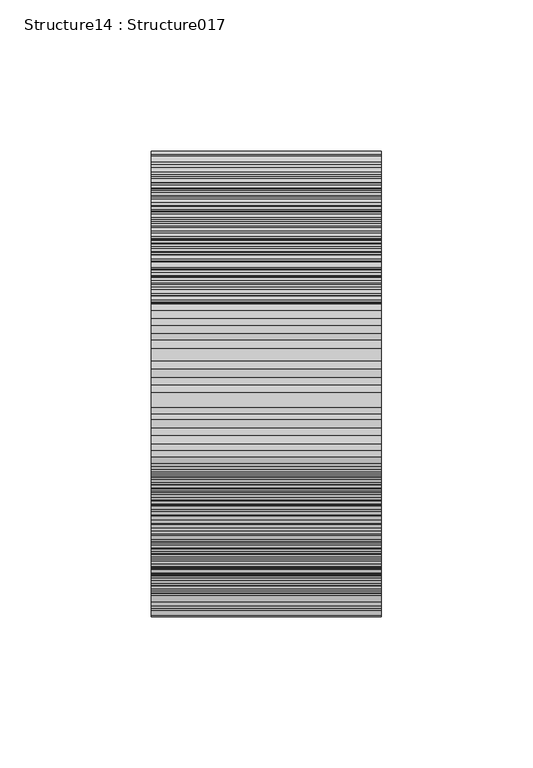
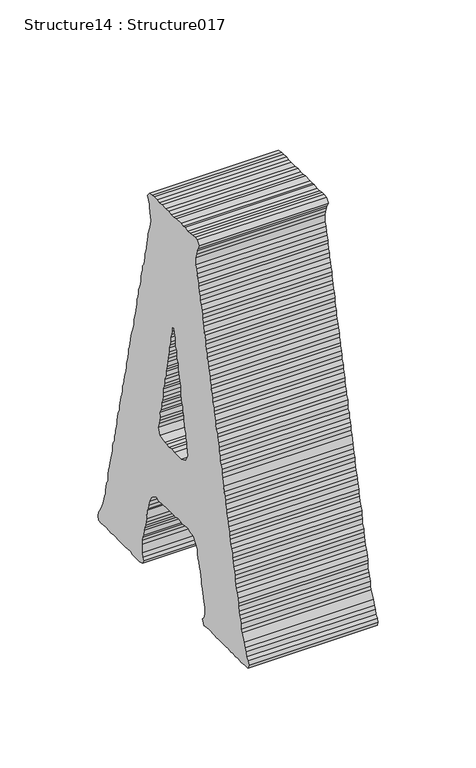
"""IFC4 building model written with IfcOpenShell, lengths in millimetres: proxy geometry, Structure14 : Structure017."""

from ifc_helpers import new_model, si_unit, frame, origin, place, context, project, spatial, polyline, outline, extrude, source, transform, mapped, element, save


def structure14_structure017_488298b9(model_context):
    return source(origin(), model_context, "Body", "SweptSolid", [
        extrude(outline(polyline([(2.1653931, 0.0), (4.9551582, -1.2411193), (7.1205514, -1.549493), (9.8959144, -1.8578666), (12.3790002, -2.7906123), (14.2258535, -3.0981388), (17.0249376, -4.0215654), (19.4987044, -4.0215654), (22.2740675, -4.9543111), (24.4394606, -5.5710584), (27.2292257, -6.1861114), (29.3937717, -6.8121777), (31.8616083, -7.1197042), (33.7101559, -8.0431309), (36.8159193, -8.3557404), (38.9813125, -8.3557404), (41.7583699, -8.9758765), (43.3112516, -9.9009975), (46.4093904, -10.5211336), (48.2664099, -11.1412697), (50.7384823, -11.758017), (53.207166, -11.758017), (55.371712, -12.3781531), (58.1614771, -13.3015797), (60.6428686, -14.2300895), (63.419926, -14.2300895), (65.2676265, -15.1585992), (68.3750842, -15.7795824), (70.2219375, -15.7795824), (72.7041762, -16.7080922), (75.1770958, -17.0198546), (77.9524588, -17.6366019), (80.1322541, -18.5642645), (84.4621932, -18.5642645), (86.9291825, -17.9432812), (89.4029494, -17.3231452), (91.2591217, -16.3997185), (93.7311941, -15.1585992), (96.2142799, -17.3231452), (96.5226536, -19.4885383), (96.5226536, -21.6581674), (95.9109893, -24.4428494), (95.9109893, -26.9149218), (96.5226536, -29.7012982), (96.2142799, -31.5532346), (96.5226536, -33.7237108), (96.5226536, -38.673786), (95.9109893, -41.1407754), (95.9109893, -43.6187781), (96.5226536, -46.4085432), (96.2142799, -49.1847535), (96.2142799, -53.2063189), (95.9109893, -55.996084), (96.5226536, -58.16063), (96.5226536, -60.9410761), (96.2142799, -63.1064692), (95.9109893, -65.8911513), (93.4245148, -67.7490179), (91.2591217, -66.5172176), (89.0945757, -65.8911513), (87.2375562, -65.584472), (84.4621932, -64.9634887), (79.8094783, -64.0392149), (77.6457795, -64.6610453), (74.8687221, -65.2710152), (69.9135639, -67.1280347), (68.3750842, -67.1280347), (65.5853191, -67.7490179), (63.1166354, -68.369154), (60.3268703, -68.6775277), (57.8437845, -69.2934278), (55.371712, -70.538783), (53.5155397, -70.538783), (50.7384823, -70.8429208), (48.2664099, -71.4630569), (46.4093904, -72.6990931), (43.6196253, -72.6990931), (41.1467056, -73.6276028), (38.9813125, -74.2477389), (36.5134759, -74.2477389), (33.7101559, -74.8636391), (31.2507912, -75.792996), (29.085398, -76.7215057), (27.2292257, -77.028185), (24.4394606, -77.3416418), (22.2740675, -78.2693043), (19.4987044, -78.2693043), (17.0249376, -79.1935782), (14.8510727, -79.5061878), (12.0748624, -80.1263238), (7.7322156, -81.6715809), (4.9551582, -81.6715809), (2.7906123, -82.291717), (0.3176926, -82.90677), (-2.4720725, -84.1478893), (-4.3282448, -84.4562629), (-6.8020116, -85.0721631), (-9.283403, -85.3847727), (-12.0604605, -86.3132824), (-13.9217158, -86.9283354), (-16.7063979, -86.9283354), (-19.4826081, -87.8568451), (-21.3438635, -88.1703019), (-24.1344758, -89.0937285), (-26.5929933, -89.4063381), (-29.0752319, -89.7147118), (-30.9322514, -90.3348478), (-33.4136429, -91.2582745), (-36.4982268, -91.5717313), (-38.9711464, -92.1918673), (-40.5240281, -93.115294), (-43.3002383, -93.115294), (-46.0908506, -93.7362772), (-48.2553966, -94.6605511), (-51.0409258, -95.2806871), (-52.9021812, -95.9008232), (-55.0531722, -96.5167233), (-57.5354109, -96.5167233), (-60.6327025, -97.7586898), (-63.1013862, -98.3737428), (-65.2794871, -98.6821165), (-67.7524067, -98.6821165), (-69.6094262, -99.3022526), (-72.6931629, -100.2349982), (-74.5501824, -100.539136), (-77.032421, -101.4718816), (-79.8128671, -101.4718816), (-81.9782603, -102.7036819), (-84.1428062, -103.323818), (-86.6106428, -103.323818), (-89.386853, -103.9439541), (-92.1910202, -104.8673807), (-94.3420113, -105.493447), (-96.2032666, -106.1093472), (-98.9887958, -106.4168737), (-101.4617155, -107.3453834), (-104.2514806, -107.9655195), (-106.7193172, -107.9655195), (-108.8982652, -108.2696573), (-111.0492563, -109.5150125), (-113.8390214, -110.1309126), (-116.311941, -110.74766), (-118.476487, -110.74766), (-120.6503519, -111.6804056), (-125.8994818, -113.2239683), (-128.0784298, -114.147395), (-129.9261303, -115.0809878), (-132.7116595, -116.9329242), (-134.2560694, -117.5589905), (-137.0314325, -118.4824172), (-139.2061446, -117.8656699), (-139.5136711, -114.7692254), (-139.2061446, -112.9113588), (-138.8884519, -110.1309126), (-139.5136711, -107.6588402), (-139.5136711, -104.8673807), (-138.8884519, -102.3953083), (-138.8884519, -100.2349982), (-139.2061446, -97.7586898), (-139.2061446, -95.5932967), (-139.5136711, -92.4951579), (-139.5136711, -90.3348478), (-139.2061446, -87.8568451), (-138.8884519, -85.0721631), (-139.5136711, -82.90677), (-139.5136711, -75.792996), (-138.8884519, -73.0066196), (-136.7374609, -71.7714306), (-134.8762055, -72.6990931), (-132.4083689, -73.3192292), (-127.1363652, -73.3192292), (-124.6634456, -73.3192292), (-122.4988996, -72.6990931), (-120.6503519, -71.7714306), (-117.5437413, -71.4630569), (-115.3791954, -70.8429208), (-113.2138022, -69.9135639), (-111.0492563, -69.2934278), (-108.5805725, -68.6775277), (-103.0145972, -68.0607803), (-101.4617155, -67.4414914), (-98.9887958, -66.5172176), (-95.8957401, -65.8911513), (-92.8018373, -64.3475886), (-90.9405819, -62.1830426), (-89.0928814, -58.7773773), (-89.7045457, -56.3044577), (-89.7045457, -51.3543825), (-89.386853, -48.2604796), (-89.386853, -41.7668417), (-89.7045457, -38.9762294), (-89.0928814, -36.8167666), (-89.386853, -34.3429997), (-89.7045457, -31.8666914), (-89.386853, -29.7012982), (-89.0928814, -26.6082425), (-89.7045457, -24.7512231), (-90.6372913, -21.04142), (-92.4943108, -19.1801646), (-95.8957401, -16.7080922), (-98.6719504, -16.7080922), (-101.4617155, -16.0862617), (-103.0145972, -15.1585992), (-106.0991811, -14.8544614), (-107.9697554, -13.6141893), (-110.7459657, -12.9982891), (-112.6029851, -12.6865267), (-115.0759048, -12.6865267), (-117.5437413, -11.4445602), (-120.0302159, -11.1412697), (-122.4988996, -10.8337432), (-124.6634456, -9.9009975), (-127.7607372, -8.9758765), (-131.7831498, -9.2800143), (-134.8762055, -10.208524), (-136.4206154, -11.758017), (-139.5136711, -9.9009975), (-139.2061446, -7.1197042), (-138.8884519, -4.6425487), (-138.8884519, 0.3075265), (-139.2061446, 2.7804461), (-139.2061446, 5.2525186), (-138.8884519, 7.4229948), (-139.2061446, 9.5875408), (-139.2061446, 12.6805965), (-138.8884519, 14.5333801), (-139.2061446, 17.6315188), (-138.8884519, 19.4876911), (-139.5136711, 21.9648467), (-138.8884519, 24.74614), (-139.5136711, 27.5316692), (-139.2061446, 29.6962152), (-138.8884519, 32.1733707), (-138.8884519, 34.6420544), (-136.4206154, 35.5748001), (-134.2560694, 34.954664), (-132.7116595, 33.405171), (-129.9261303, 32.790118), (-128.0784298, 31.8616083), (-125.2742626, 30.6196418), (-120.6503519, 28.4550958), (-118.7797776, 27.8400429), (-115.7002768, 27.5316692), (-113.2138022, 26.9115331), (-111.0492563, 26.2947858), (-109.2015558, 25.3620401), (-106.0991811, 25.0536665), (-104.2514806, 25.0536665), (-101.4617155, 24.4377663), (-98.6719504, 23.5092566), (-96.5201121, 22.5765109), (-94.3420113, 21.9648467), (-91.565801, 21.6530843), (-89.0928814, 21.3396275), (-86.9190164, 21.0329482), (-84.7629423, 19.7960648), (-81.6563317, 19.4876911), (-79.5053406, 19.1750816), (-77.032421, 18.8675551), (-74.858556, 17.9441284), (-72.3856364, 17.0113828), (-69.6094262, 16.3946354), (-68.0556973, 15.7744994), (-65.5827776, 15.7744994), (-62.7980956, 14.8459896), (-60.0074833, 14.5333801), (-58.151311, 13.922563), (-55.6783914, 12.9889702), (-53.5223172, 12.6805965), (-50.7232331, 11.7529339), (-48.2553966, 11.7529339), (-46.0908506, 11.1311035), (-43.617931, 10.5160505), (-40.8273187, 9.9009975), (-36.1949362, 8.659031), (-33.7220165, 8.0422837), (-31.2397779, 8.0422837), (-29.0752319, 7.1095381), (-26.910686, 6.1861114), (-23.8125472, 6.1861114), (-21.9690826, 4.9458393), (-19.4826081, 4.9458393), (-16.7063979, 4.6425487), (-14.2250064, 3.4005822), (-12.0604605, 3.4005822), (-9.9094694, 2.164546), (-6.8020116, 1.8570195), (-4.6366185, 1.8570195), (-1.8612554, 0.6201361), (0.0, 0.0), (2.1653931, 0.0)]), holes=[polyline([(-49.7947234, -33.0976445), (-49.7947234, -40.2173487), (-49.5007518, -42.9977949), (-50.1124161, -45.7884072), (-49.5007518, -47.9521059), (-49.7947234, -50.1174991), (-48.2553966, -54.7558119), (-44.2423029, -56.3044577), (-41.1450113, -55.6843216), (-38.9711464, -55.0624912), (-36.8150722, -54.4525213), (-33.7220165, -54.7558119), (-31.5430685, -53.5189285), (-29.0752319, -53.2063189), (-26.910686, -52.8987924), (-24.7452928, -51.9745186), (-22.2639014, -51.6627562), (-19.7909818, -51.6627562), (-17.0147715, -51.3543825), (-15.1535162, -50.4301087), (-12.6848324, -49.8099726), (-10.203441, -49.8099726), (-7.4221477, -48.5739364), (-4.6366185, -48.5739364), (-2.4720725, -47.6403436), (-0.6099699, -47.3319699), (2.4737668, -47.0193603), (4.9551582, -46.4085432), (7.423842, -45.7884072), (9.5892351, -45.4757976), (12.0748624, -45.4757976), (14.5435462, -44.2389142), (16.7089393, -43.9305405), (19.4987044, -43.9305405), (21.9563748, -42.9977949), (24.1353229, -42.3869778), (26.300716, -42.3869778), (26.6040066, -41.4542322), (24.1353229, -40.838332), (21.6496955, -39.9089751), (19.1810118, -39.5972127), (16.4048016, -39.5972127), (14.5435462, -38.3654124), (11.7537811, -38.0519556), (9.8959144, -38.0519556), (7.423842, -36.8167666), (4.3307863, -36.5083929), (2.1653931, -36.1957833), (0.0, -35.5756472), (-2.4720725, -35.2672736), (-5.2567545, -34.3429997), (-10.203441, -34.0303902), (-12.6848324, -33.4102541), (-15.1535162, -33.0976445), (-16.7063979, -32.1733707), (-19.4826081, -32.1733707), (-21.9690826, -30.9373345), (-24.4377663, -30.9373345), (-26.5929933, -30.3171984), (-29.3920774, -30.0088247), (-31.2397779, -29.0752319), (-34.0159881, -29.0752319), (-36.8150722, -28.1518052), (-38.6627727, -28.1518052), (-41.1450113, -27.5316692), (-44.2423029, -26.9149218), (-47.9470229, -28.7727885), (-49.7947234, -33.0976445)])]), frame((-35624.0862846, 275817.8272661, 4122.0266343), z_axis=(1.0, 0.0, 1.354250045437766e-12), x_axis=(-1.354250045437766e-12, 0.0, 1.0)), (0.0, 0.0, 1.0), 76.2),
    ])


if __name__ == "__main__":
    model = new_model("IFC4")
    model_context = context("Model", 3, world=origin())
    ifc_project = project(units=[si_unit("LENGTHUNIT", "METRE", prefix="MILLI")], contexts=[model_context])
    site = spatial("IfcSite", under=ifc_project)
    building = spatial("IfcBuilding", under=site)
    placement = place(None, origin())
    structure14_structure017_shape = structure14_structure017_488298b9(model_context)
    element("IfcBuildingElementProxy", 1, Name="Structure14 : Structure017", ObjectType="Structure14 : Structure017", at=placement, inside=building, context=model_context, shape_type="MappedRepresentation", body=[
        mapped(structure14_structure017_shape, transform((0.0, 0.0, 0.0), x_axis=(1.0, 0.0, 0.0), y_axis=(0.0, 1.0, 0.0), z_axis=(0.0, 0.0, 1.0))),
    ])
    save(model, "model.ifc")

# Revit data of these elements
# Type "Structure14 : Structure017"
#   NameOverride = "Structure017"
# Element 1 (IfcBuildingElementProxy, "Structure14 : Structure017")
#   Materials on its faces: "BRUSHED ALUMINUM LETTERING"
# Materials
#   "BRUSHED ALUMINUM LETTERING": class "Unassigned", colour RGB 169 181 186, transparency 0, Cost = 0
